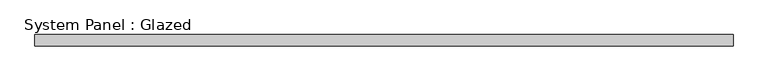
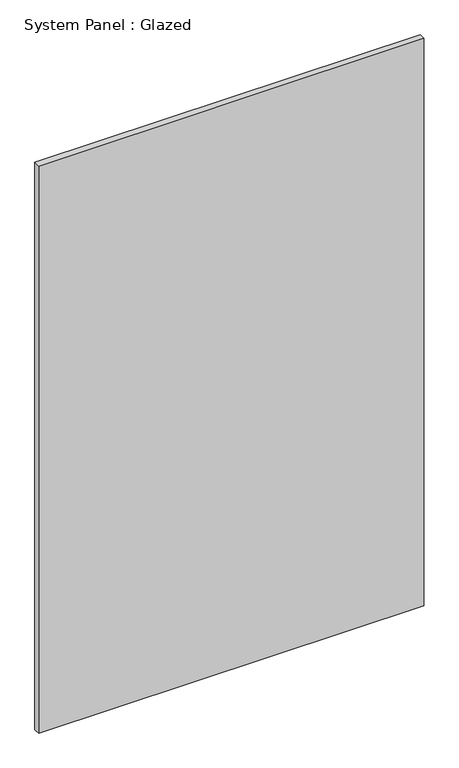
"""IFC4 building model written with IfcOpenShell, lengths in millimetres: plate geometry, System Panel : Glazed."""

from ifc_helpers import new_model, si_unit, origin, origin_with_axes, place, context, project, spatial, polyline, outline, extrude, source, transform, mapped, element, save


def system_panel_glazed_2bdc609b(model_context):
    return source(origin(), model_context, "Body", "SweptSolid", [
        extrude(outline(polyline([(769.3237049, 24.5), (-769.3237049, 24.5), (-769.3237049, 49.5), (769.3237049, 49.5), (769.3237049, 24.5)])), origin_with_axes(), (0.0, 0.0, 1.0), 2395.0),
    ])


if __name__ == "__main__":
    model = new_model("IFC4")
    model_context = context("Model", 3, world=origin())
    ifc_project = project(units=[si_unit("LENGTHUNIT", "METRE", prefix="MILLI")], contexts=[model_context])
    site = spatial("IfcSite", under=ifc_project)
    building = spatial("IfcBuilding", under=site)
    placement = place(None, origin())
    system_panel_glazed_shape = system_panel_glazed_2bdc609b(model_context)
    element("IfcPlate", 1, ObjectType="System Panel : Glazed", at=placement, inside=building, context=model_context, shape_type="MappedRepresentation", body=[
        mapped(system_panel_glazed_shape, transform((0.0, 0.0, 0.0), x_axis=(1.0, 0.0, 0.0), y_axis=(0.0, 1.0, 0.0), z_axis=(0.0, 0.0, 1.0))),
    ])
    save(model, "model.ifc")

# Revit data of these elements
# Element 1 (IfcPlate, "System Panel : Glazed")
#   Materials on its faces: "Glass"
# Materials
#   "Glass": class "Glass", colour RGB 218 227 224, transparency 0.85, Description = "Soda Lime Glass", Cost = 0
